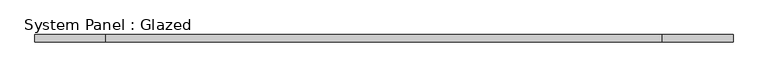
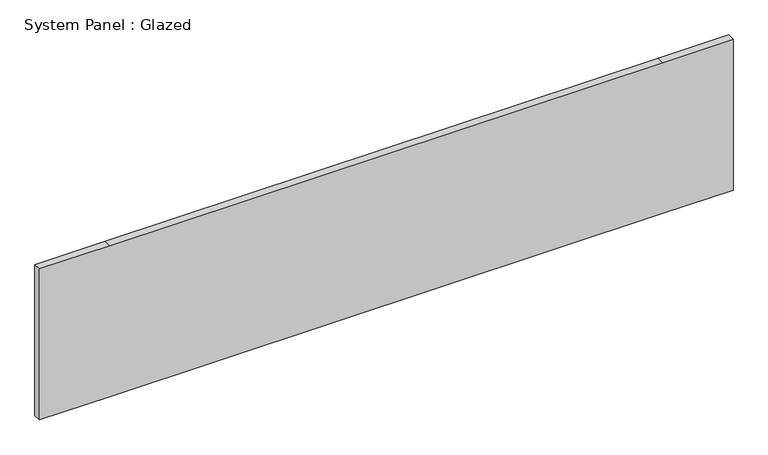
"""IFC4 building model written with IfcOpenShell, lengths in millimetres: plate geometry, System Panel : Glazed."""

import ifcopenshell
import ifcopenshell.guid

model = None  # the IFC model being written
_history = None  # IfcOwnerHistory: only IFC2X3 demands one
_inside = {}  # id of a spatial element -> (the spatial element, [elements in it])
_under = {}  # id of a project, library or spatial element -> (it, [spatial elements below it])
_declared = {}  # id of a project -> (the project, [libraries it declares])
_typed = {}  # id of a type object -> (the type object, [elements of that type])
_made_of = {}  # id of a material, layer set ... -> (it, [elements and type objects made of it])


def new_model(schema):
    """Start an empty IFC model of exactly this schema.

    Asked for "IFC4X3", IfcOpenShell would pick the latest addendum, in which some entities
    have other attributes; the version numbers below select the first issue.
    IFC2X3 requires an IfcOwnerHistory on every rooted entity: one is made here for all.
    """
    global model, _history
    if schema == "IFC4X3":
        model = ifcopenshell.file(schema_version=(4, 3, 0, 0))
    else:
        model = ifcopenshell.file(schema=schema)
    _inside.clear()
    _under.clear()
    _declared.clear()
    _typed.clear()
    _made_of.clear()
    _history = None
    if model.schema == "IFC2X3":
        org = make("IfcOrganization", Name="unknown")
        user = make(
            "IfcPersonAndOrganization",
            ThePerson=make("IfcPerson", FamilyName="unknown"),
            TheOrganization=org,
        )
        app = make(
            "IfcApplication",
            ApplicationDeveloper=org,
            Version="unknown",
            ApplicationFullName="unknown",
            ApplicationIdentifier="unknown",
        )
        _history = make(
            "IfcOwnerHistory",
            OwningUser=user,
            OwningApplication=app,
            ChangeAction="ADDED",
            CreationDate=0,
        )
    return model


def make(cls, **values):
    """One entity of the class cls with the attributes given. An attribute that is None is left unset."""
    return model.create_entity(
        cls, **{name: value for name, value in values.items() if value is not None}
    )


def rooted(cls, **values):
    """An entity with a GlobalId (a new one), such as an element, a storey or a relation."""
    return make(cls, GlobalId=ifcopenshell.guid.new(), OwnerHistory=_history, **values)


def si_unit(unit_type, name, prefix=None):
    """IfcSIUnit, for example si_unit("LENGTHUNIT", "METRE", prefix="MILLI")."""
    return make("IfcSIUnit", UnitType=unit_type, Prefix=prefix, Name=name)


def assignment(units):
    """IfcUnitAssignment: the units of a project."""
    return None if units is None else make("IfcUnitAssignment", Units=units)


def point(xyz):
    """IfcCartesianPoint."""
    return None if xyz is None else make("IfcCartesianPoint", Coordinates=xyz)


def direction(xyz):
    """IfcDirection."""
    return None if xyz is None else make("IfcDirection", DirectionRatios=xyz)


def frame(location, z_axis=None, x_axis=None):
    """IfcAxis2Placement3D, a coordinate frame: its origin and axes. An axis left out is left unset."""
    return make(
        "IfcAxis2Placement3D",
        Location=point(location),
        Axis=direction(z_axis),
        RefDirection=direction(x_axis),
    )


def origin():
    """The frame at (0, 0, 0) with its axes left unset."""
    return frame((0.0, 0.0, 0.0))


def place(relative_to, where):
    """IfcLocalPlacement: puts the frame where relative to a parent placement (None: the world)."""
    return make(
        "IfcLocalPlacement", PlacementRelTo=relative_to, RelativePlacement=where
    )


def context(
    kind, dimensions, precision=None, world=None, true_north=None, identifier=None
):
    """IfcGeometricRepresentationContext, for example the 3D "Model" context."""
    return make(
        "IfcGeometricRepresentationContext",
        ContextIdentifier=identifier,
        ContextType=kind,
        CoordinateSpaceDimension=dimensions,
        Precision=precision,
        WorldCoordinateSystem=world,
        TrueNorth=true_north,
    )


def project(units=None, contexts=None):
    """IfcProject with its units and contexts."""
    return rooted(
        "IfcProject",
        Name="project",
        RepresentationContexts=contexts,
        UnitsInContext=assignment(units),
    )


def spatial(cls, under=None, at=None, **own):
    """A site, building, storey or space (cls), placed at a placement, below another one or the project."""
    s = rooted(cls, ObjectPlacement=at, **own)
    if under is not None:
        _under.setdefault(under.id(), (under, []))[1].append(s)
    return s


def polyline(points):
    """IfcPolyline through the points."""
    return make("IfcPolyline", Points=[point(p) for p in points])


def outline(outer, holes=None, kind="AREA"):
    """IfcArbitraryClosedProfileDef: a profile drawn as a closed curve; with holes, ...WithVoids."""
    if holes is None:
        return make("IfcArbitraryClosedProfileDef", ProfileType=kind, OuterCurve=outer)
    return make(
        "IfcArbitraryProfileDefWithVoids",
        ProfileType=kind,
        OuterCurve=outer,
        InnerCurves=holes,
    )


def extrude(swept, where, along, depth):
    """IfcExtrudedAreaSolid: the profile swept, set in the frame where, extruded along a direction by depth."""
    return make(
        "IfcExtrudedAreaSolid",
        SweptArea=swept,
        Position=where,
        ExtrudedDirection=direction(along),
        Depth=depth,
    )


def shape(context_of_items, identifier, shape_type, items):
    """IfcShapeRepresentation: the items that make up one representation, for example the "Body"."""
    return make(
        "IfcShapeRepresentation",
        ContextOfItems=context_of_items,
        RepresentationIdentifier=identifier,
        RepresentationType=shape_type,
        Items=items,
    )


def source(mapping_origin, context_of_items, identifier, shape_type, items):
    """IfcRepresentationMap: a shape defined once, which mapped items show again and again."""
    return make(
        "IfcRepresentationMap",
        MappingOrigin=mapping_origin,
        MappedRepresentation=shape(context_of_items, identifier, shape_type, items),
    )


def transform(
    local_origin,
    x_axis=None,
    y_axis=None,
    z_axis=None,
    scale=None,
    scale2=None,
    scale3=None,
    uniform=True,
):
    """IfcCartesianTransformationOperator3D, or its non-uniform kind. x_axis, y_axis, z_axis: its Axis1, 2, 3."""
    if uniform:
        return make(
            "IfcCartesianTransformationOperator3D",
            Axis1=direction(x_axis),
            Axis2=direction(y_axis),
            LocalOrigin=point(local_origin),
            Scale=scale,
            Axis3=direction(z_axis),
        )
    return make(
        "IfcCartesianTransformationOperator3DnonUniform",
        Axis1=direction(x_axis),
        Axis2=direction(y_axis),
        LocalOrigin=point(local_origin),
        Scale=scale,
        Axis3=direction(z_axis),
        Scale2=scale2,
        Scale3=scale3,
    )


def mapped(mapping_source, mapping_target):
    """IfcMappedItem: shows the shape of a source again, moved by a transform."""
    return make(
        "IfcMappedItem", MappingSource=mapping_source, MappingTarget=mapping_target
    )


def made_of(thing, what):
    """Note that an element or type object is made of a material, layer set ...; save() writes the relation."""
    if what is not None:
        _made_of.setdefault(what.id(), (what, []))[1].append(thing)
    return thing


def element(
    cls,
    number,
    at=None,
    inside=None,
    cuts=None,
    type_object=None,
    material=None,
    context=None,
    identifier="Body",
    shape_type=None,
    held_by="IfcProductDefinitionShape",
    body=None,
    shapes=None,
    **own,
):
    """One element of the class cls, such as IfcWall. Its Tag is "e" and its number.

    at: its placement. inside: the storey or other place that contains it. cuts: it is an
    opening in that element (IfcRelVoidsElement). A single representation is given by context,
    identifier, shape_type and body (its items); several are given by shapes. held_by: the class
    of the entity that holds the representations. save() writes the other relations.
    """
    e = rooted(cls, Tag="e%d" % number, ObjectPlacement=at, **own)
    if body is not None:
        shapes = [shape(context, identifier, shape_type, body)]
    if shapes is not None:
        e.Representation = make(held_by, Representations=shapes)
    if inside is not None:
        _inside.setdefault(inside.id(), (inside, []))[1].append(e)
    if cuts is not None:
        rooted(
            "IfcRelVoidsElement", RelatingBuildingElement=cuts, RelatedOpeningElement=e
        )
    if type_object is not None:
        _typed.setdefault(type_object.id(), (type_object, []))[1].append(e)
    return made_of(e, material)


def aggregate(whole, parts):
    """IfcRelAggregates: a whole, such as a stair, and the parts it consists of."""
    return rooted("IfcRelAggregates", RelatingObject=whole, RelatedObjects=parts)


def save(model, path):
    """Write the relations noted so far, then the file.

    IfcRelAggregates (storeys below a building ...), IfcRelContainedInSpatialStructure (elements
    in a storey), IfcRelDefinesByType, IfcRelAssociatesMaterial and IfcRelDeclares: one each for
    every whole, place, type object, material and project.
    """
    for whole, parts in _under.values():
        aggregate(whole, parts)
    for where, things in _inside.values():
        rooted(
            "IfcRelContainedInSpatialStructure",
            RelatedElements=things,
            RelatingStructure=where,
        )
    for kind, things in _typed.values():
        rooted("IfcRelDefinesByType", RelatedObjects=things, RelatingType=kind)
    for what, things in _made_of.values():
        rooted("IfcRelAssociatesMaterial", RelatedObjects=things, RelatingMaterial=what)
    for by, libraries in _declared.values():
        rooted("IfcRelDeclares", RelatingContext=by, RelatedDefinitions=libraries)
    model.write(path)


def system_panel_glazed_7ab8f380(model_context):
    return source(origin(), model_context, "Body", "SweptSolid", [
        extrude(outline(polyline([(0.0, -1187.45), (0.0, -946.15), (0.0, 946.15), (0.0, 1187.45), (546.1, 1187.45), (546.1, 946.15), (546.1, -946.15), (546.1, -1187.45), (0.0, -1187.45)])), frame((0.0, -44.45, 0.0), z_axis=(0.0, 1.0, 0.0), x_axis=(0.0, 0.0, 1.0)), (0.0, 0.0, 1.0), 25.4),
    ])


if __name__ == "__main__":
    model = new_model("IFC4")
    model_context = context("Model", 3, world=origin())
    ifc_project = project(units=[si_unit("LENGTHUNIT", "METRE", prefix="MILLI")], contexts=[model_context])
    site = spatial("IfcSite", under=ifc_project)
    building = spatial("IfcBuilding", under=site)
    placement = place(None, origin())
    system_panel_glazed_shape = system_panel_glazed_7ab8f380(model_context)
    element("IfcPlate", 1, ObjectType="System Panel : Glazed", at=placement, inside=building, context=model_context, shape_type="MappedRepresentation", body=[
        mapped(system_panel_glazed_shape, transform((0.0, 0.0, 0.0), x_axis=(1.0, 0.0, 0.0), y_axis=(0.0, 1.0, 0.0), z_axis=(0.0, 0.0, 1.0))),
    ])
    save(model, "model.ifc")

# Revit data of these elements
# Element 1 (IfcPlate, "System Panel : Glazed")
#   Materials on its faces: "Glass"
# Materials
#   "Glass": class "Glass", colour RGB 0 128 192, transparency 0.75
